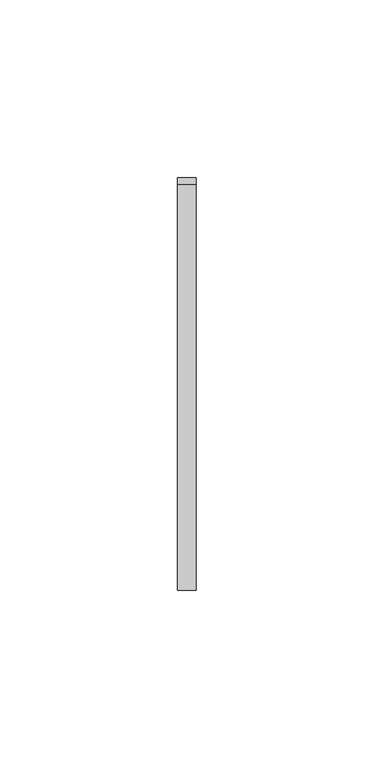
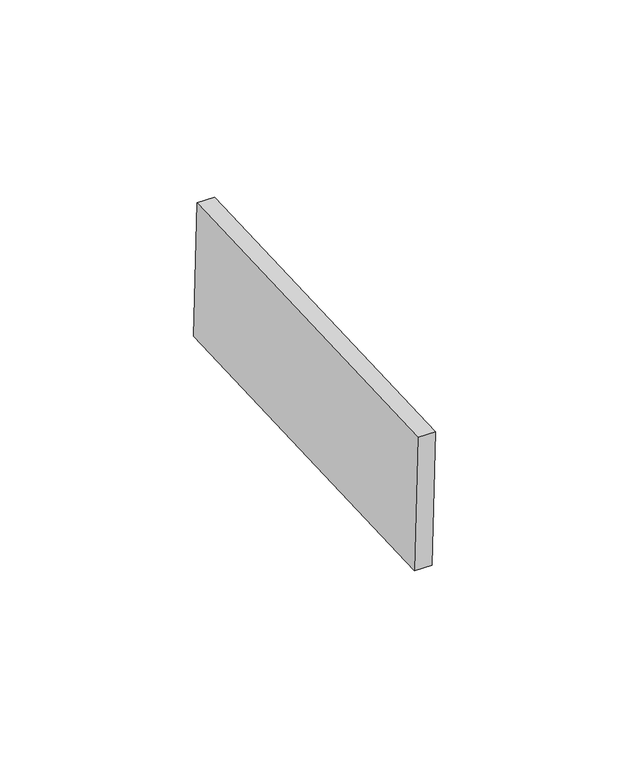
"""IFC4 building model written with IfcOpenShell, lengths in millimetres: proxy geometry, Inner panel:Inner panel:1:Inner panel:1 : Inner panel:Inner panel:300324:2:Inner panel:1:Inner panel:1 : Inner panel:Inner panel:300324:2 : Inner panel:Inner panel:1:Inner panel:1 : Inner panel:Inner panel:300324:300043:79 : Inner panel:Inner panel:1:Inner panel:1 : Inner panel:Inner panel:300324:2:Inner panel:1:Inner panel:1 : Inner panel:Inner panel:300324:2 : Inner panel:Inner panel:1:Inner panel:1 : Inner panel:Inner panel:300324:300043:308120."""

from ifc_helpers import new_model, si_unit, frame, origin, place, context, project, spatial, polyline, outline, extrude, source, transform, mapped, element, save


def generic_models_0da32b7d(model_context):
    return source(origin(), model_context, "Body", "SweptSolid", [
        extrude(outline(polyline([(0.0, -114.3), (0.0, 0.0), (5.2138089, 0.0), (5.2138089, -114.3), (0.0, -114.3)])), frame((591904.595117, -578297.797364, 3981.6641254), z_axis=(0.0, -0.04163054471216399, 0.9991330730923527), x_axis=(-1.0, 0.0, 0.0)), (0.0, 0.0, 1.0), 43.2233908),
    ])


if __name__ == "__main__":
    model = new_model("IFC4")
    model_context = context("Model", 3, world=origin())
    ifc_project = project(units=[si_unit("LENGTHUNIT", "METRE", prefix="MILLI")], contexts=[model_context])
    site = spatial("IfcSite", under=ifc_project)
    building = spatial("IfcBuilding", under=site)
    placement = place(None, origin())
    generic_models_shape = generic_models_0da32b7d(model_context)
    element("IfcBuildingElementProxy", 1, Name="Inner panel:Inner panel:1:Inner panel:1 : Inner panel:Inner panel:300324:2:Inner panel:1:Inner panel:1 : Inner panel:Inner panel:300324:2 : Inner panel:Inner panel:1:Inner panel:1 : Inner panel:Inner panel:300324:300043:79 : Inner panel:Inner panel:1:Inner panel:1 : Inner panel:Inner panel:300324:2:Inner panel:1:Inner panel:1 : Inner panel:Inner panel:300324:2 : Inner panel:Inner panel:1:Inner panel:1 : Inner panel:Inner panel:300324:300043:308120", ObjectType="Inner panel:Inner panel:1:Inner panel:1 : Inner panel:Inner panel:300324:2:Inner panel:1:Inner panel:1 : Inner panel:Inner panel:300324:2 : Inner panel:Inner panel:1:Inner panel:1 : Inner panel:Inner panel:300324:300043:79 : Inner panel:Inner panel:1:Inner panel:1 : Inner panel:Inner panel:300324:2:Inner panel:1:Inner panel:1 : Inner panel:Inner panel:300324:2 : Inner panel:Inner panel:1:Inner panel:1 : Inner panel:Inner panel:300324:300043:308120", at=placement, inside=building, context=model_context, shape_type="MappedRepresentation", body=[
        mapped(generic_models_shape, transform((0.0, 0.0, 0.0), x_axis=(1.0, 0.0, 0.0), y_axis=(0.0, 1.0, 0.0), z_axis=(0.0, 0.0, 1.0))),
    ])
    save(model, "model.ifc")

# Revit data of these elements
# Type "Inner panel:Inner panel:1:Inner panel:1 : Inner panel:Inner panel:300324:2:Inner panel:1:Inner panel:1 : Inner panel:Inner panel:300324:2 : Inner panel:Inner panel:1:Inner panel:1 : Inner panel:Inner panel:300324:300043:79 : Inner panel:Inner panel:1:Inner panel:1 : Inner panel:Inner panel:300324:2:Inner panel:1:Inner panel:1 : Inner panel:Inner panel:300324:2 : Inner panel:Inner panel:1:Inner panel:1 : Inner panel:Inner panel:300324:300043:308120"
#   NameOverride = "Inner panel:Inner panel:1:Inner panel:1 : Inner panel:Inner panel:300324:2:Inner panel:1:Inner panel:1 : Inner panel:Inner panel:300324:2 : Inner panel:Inner panel:1:Inner panel:1 : Inner panel:Inner panel:300324:300043:308120"
#   ObjectTypeOverride = "Inner panel:1:Inner panel:1 : Inner panel:Inner panel:300324:2 : Inner panel:Inner panel:1:Inner panel:1 : Inner panel:Inner panel:300324:300043"
#   Reference = "Inner panel"
#   Tag = "308120"
# Element 1 (IfcBuildingElementProxy, "Inner panel:Inner panel:1:Inner panel:1 : Inner panel:Inner panel:300324:2:Inner panel:1:Inner panel:1 : Inner panel:Inner panel:300324:2 : Inner panel:Inner panel:1:Inner panel:1 : Inner panel:Inner panel:300324:300043:79 : Inner panel:Inner panel:1:Inner panel:1 : Inner panel:Inner panel:300324:2:Inner panel:1:Inner panel:1 : Inner panel:Inner panel:300324:2 : Inner panel:Inner panel:1:Inner panel:1 : Inner panel:Inner panel:300324:300043:308120")
#   Materials on its faces: "SLIDING CLIP"
# Materials
#   "SLIDING CLIP": class "Generic", colour RGB 120 120 120, transparency 0, Cost = 0
